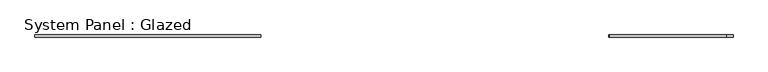
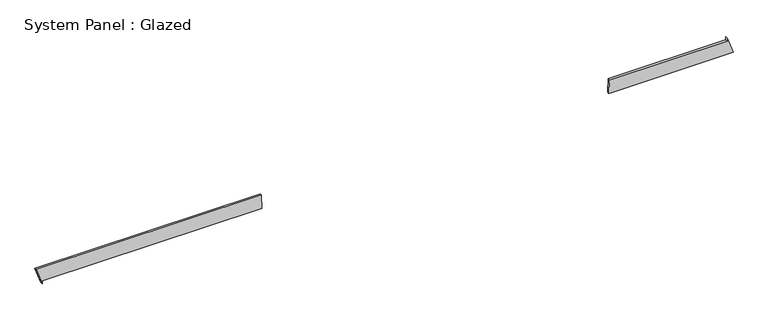
"""IFC4 building model written with IfcOpenShell, lengths in millimetres: plate geometry, System Panel : Glazed."""

import ifcopenshell
import ifcopenshell.guid

model = None  # the IFC model being written
_history = None  # IfcOwnerHistory: only IFC2X3 demands one
_inside = {}  # id of a spatial element -> (the spatial element, [elements in it])
_under = {}  # id of a project, library or spatial element -> (it, [spatial elements below it])
_declared = {}  # id of a project -> (the project, [libraries it declares])
_typed = {}  # id of a type object -> (the type object, [elements of that type])
_made_of = {}  # id of a material, layer set ... -> (it, [elements and type objects made of it])


def new_model(schema):
    """Start an empty IFC model of exactly this schema.

    Asked for "IFC4X3", IfcOpenShell would pick the latest addendum, in which some entities
    have other attributes; the version numbers below select the first issue.
    IFC2X3 requires an IfcOwnerHistory on every rooted entity: one is made here for all.
    """
    global model, _history
    if schema == "IFC4X3":
        model = ifcopenshell.file(schema_version=(4, 3, 0, 0))
    else:
        model = ifcopenshell.file(schema=schema)
    _inside.clear()
    _under.clear()
    _declared.clear()
    _typed.clear()
    _made_of.clear()
    _history = None
    if model.schema == "IFC2X3":
        org = make("IfcOrganization", Name="unknown")
        user = make(
            "IfcPersonAndOrganization",
            ThePerson=make("IfcPerson", FamilyName="unknown"),
            TheOrganization=org,
        )
        app = make(
            "IfcApplication",
            ApplicationDeveloper=org,
            Version="unknown",
            ApplicationFullName="unknown",
            ApplicationIdentifier="unknown",
        )
        _history = make(
            "IfcOwnerHistory",
            OwningUser=user,
            OwningApplication=app,
            ChangeAction="ADDED",
            CreationDate=0,
        )
    return model


def make(cls, **values):
    """One entity of the class cls with the attributes given. An attribute that is None is left unset."""
    return model.create_entity(
        cls, **{name: value for name, value in values.items() if value is not None}
    )


def rooted(cls, **values):
    """An entity with a GlobalId (a new one), such as an element, a storey or a relation."""
    return make(cls, GlobalId=ifcopenshell.guid.new(), OwnerHistory=_history, **values)


def si_unit(unit_type, name, prefix=None):
    """IfcSIUnit, for example si_unit("LENGTHUNIT", "METRE", prefix="MILLI")."""
    return make("IfcSIUnit", UnitType=unit_type, Prefix=prefix, Name=name)


def assignment(units):
    """IfcUnitAssignment: the units of a project."""
    return None if units is None else make("IfcUnitAssignment", Units=units)


def point(xyz):
    """IfcCartesianPoint."""
    return None if xyz is None else make("IfcCartesianPoint", Coordinates=xyz)


def direction(xyz):
    """IfcDirection."""
    return None if xyz is None else make("IfcDirection", DirectionRatios=xyz)


def frame(location, z_axis=None, x_axis=None):
    """IfcAxis2Placement3D, a coordinate frame: its origin and axes. An axis left out is left unset."""
    return make(
        "IfcAxis2Placement3D",
        Location=point(location),
        Axis=direction(z_axis),
        RefDirection=direction(x_axis),
    )


def origin():
    """The frame at (0, 0, 0) with its axes left unset."""
    return frame((0.0, 0.0, 0.0))


def place(relative_to, where):
    """IfcLocalPlacement: puts the frame where relative to a parent placement (None: the world)."""
    return make(
        "IfcLocalPlacement", PlacementRelTo=relative_to, RelativePlacement=where
    )


def context(
    kind, dimensions, precision=None, world=None, true_north=None, identifier=None
):
    """IfcGeometricRepresentationContext, for example the 3D "Model" context."""
    return make(
        "IfcGeometricRepresentationContext",
        ContextIdentifier=identifier,
        ContextType=kind,
        CoordinateSpaceDimension=dimensions,
        Precision=precision,
        WorldCoordinateSystem=world,
        TrueNorth=true_north,
    )


def project(units=None, contexts=None):
    """IfcProject with its units and contexts."""
    return rooted(
        "IfcProject",
        Name="project",
        RepresentationContexts=contexts,
        UnitsInContext=assignment(units),
    )


def spatial(cls, under=None, at=None, **own):
    """A site, building, storey or space (cls), placed at a placement, below another one or the project."""
    s = rooted(cls, ObjectPlacement=at, **own)
    if under is not None:
        _under.setdefault(under.id(), (under, []))[1].append(s)
    return s


def polyline(points):
    """IfcPolyline through the points."""
    return make("IfcPolyline", Points=[point(p) for p in points])


def outline(outer, holes=None, kind="AREA"):
    """IfcArbitraryClosedProfileDef: a profile drawn as a closed curve; with holes, ...WithVoids."""
    if holes is None:
        return make("IfcArbitraryClosedProfileDef", ProfileType=kind, OuterCurve=outer)
    return make(
        "IfcArbitraryProfileDefWithVoids",
        ProfileType=kind,
        OuterCurve=outer,
        InnerCurves=holes,
    )


def extrude(swept, where, along, depth):
    """IfcExtrudedAreaSolid: the profile swept, set in the frame where, extruded along a direction by depth."""
    return make(
        "IfcExtrudedAreaSolid",
        SweptArea=swept,
        Position=where,
        ExtrudedDirection=direction(along),
        Depth=depth,
    )


def shape(context_of_items, identifier, shape_type, items):
    """IfcShapeRepresentation: the items that make up one representation, for example the "Body"."""
    return make(
        "IfcShapeRepresentation",
        ContextOfItems=context_of_items,
        RepresentationIdentifier=identifier,
        RepresentationType=shape_type,
        Items=items,
    )


def source(mapping_origin, context_of_items, identifier, shape_type, items):
    """IfcRepresentationMap: a shape defined once, which mapped items show again and again."""
    return make(
        "IfcRepresentationMap",
        MappingOrigin=mapping_origin,
        MappedRepresentation=shape(context_of_items, identifier, shape_type, items),
    )


def transform(
    local_origin,
    x_axis=None,
    y_axis=None,
    z_axis=None,
    scale=None,
    scale2=None,
    scale3=None,
    uniform=True,
):
    """IfcCartesianTransformationOperator3D, or its non-uniform kind. x_axis, y_axis, z_axis: its Axis1, 2, 3."""
    if uniform:
        return make(
            "IfcCartesianTransformationOperator3D",
            Axis1=direction(x_axis),
            Axis2=direction(y_axis),
            LocalOrigin=point(local_origin),
            Scale=scale,
            Axis3=direction(z_axis),
        )
    return make(
        "IfcCartesianTransformationOperator3DnonUniform",
        Axis1=direction(x_axis),
        Axis2=direction(y_axis),
        LocalOrigin=point(local_origin),
        Scale=scale,
        Axis3=direction(z_axis),
        Scale2=scale2,
        Scale3=scale3,
    )


def mapped(mapping_source, mapping_target):
    """IfcMappedItem: shows the shape of a source again, moved by a transform."""
    return make(
        "IfcMappedItem", MappingSource=mapping_source, MappingTarget=mapping_target
    )


def made_of(thing, what):
    """Note that an element or type object is made of a material, layer set ...; save() writes the relation."""
    if what is not None:
        _made_of.setdefault(what.id(), (what, []))[1].append(thing)
    return thing


def element(
    cls,
    number,
    at=None,
    inside=None,
    cuts=None,
    type_object=None,
    material=None,
    context=None,
    identifier="Body",
    shape_type=None,
    held_by="IfcProductDefinitionShape",
    body=None,
    shapes=None,
    **own,
):
    """One element of the class cls, such as IfcWall. Its Tag is "e" and its number.

    at: its placement. inside: the storey or other place that contains it. cuts: it is an
    opening in that element (IfcRelVoidsElement). A single representation is given by context,
    identifier, shape_type and body (its items); several are given by shapes. held_by: the class
    of the entity that holds the representations. save() writes the other relations.
    """
    e = rooted(cls, Tag="e%d" % number, ObjectPlacement=at, **own)
    if body is not None:
        shapes = [shape(context, identifier, shape_type, body)]
    if shapes is not None:
        e.Representation = make(held_by, Representations=shapes)
    if inside is not None:
        _inside.setdefault(inside.id(), (inside, []))[1].append(e)
    if cuts is not None:
        rooted(
            "IfcRelVoidsElement", RelatingBuildingElement=cuts, RelatedOpeningElement=e
        )
    if type_object is not None:
        _typed.setdefault(type_object.id(), (type_object, []))[1].append(e)
    return made_of(e, material)


def aggregate(whole, parts):
    """IfcRelAggregates: a whole, such as a stair, and the parts it consists of."""
    return rooted("IfcRelAggregates", RelatingObject=whole, RelatedObjects=parts)


def save(model, path):
    """Write the relations noted so far, then the file.

    IfcRelAggregates (storeys below a building ...), IfcRelContainedInSpatialStructure (elements
    in a storey), IfcRelDefinesByType, IfcRelAssociatesMaterial and IfcRelDeclares: one each for
    every whole, place, type object, material and project.
    """
    for whole, parts in _under.values():
        aggregate(whole, parts)
    for where, things in _inside.values():
        rooted(
            "IfcRelContainedInSpatialStructure",
            RelatedElements=things,
            RelatingStructure=where,
        )
    for kind, things in _typed.values():
        rooted("IfcRelDefinesByType", RelatedObjects=things, RelatingType=kind)
    for what, things in _made_of.values():
        rooted("IfcRelAssociatesMaterial", RelatedObjects=things, RelatingMaterial=what)
    for by, libraries in _declared.values():
        rooted("IfcRelDeclares", RelatingContext=by, RelatedDefinitions=libraries)
    model.write(path)


def system_panel_glazed_22199b68(model_context):
    return source(origin(), model_context, "Body", "SweptSolid", [
        extrude(outline(polyline([(35.3553391, 2592.9093212), (35.3553391, 4027.1398136), (235.0472205, 3956.767991), (199.6918814, 3956.7680004), (199.6915206, 2596.4691848), (35.3553391, 2592.9093212)])), frame((0.0, -49.5, 0.0), z_axis=(0.0, 1.0, 0.0), x_axis=(0.0, 0.0, 1.0)), (0.0, 0.0, 1.0), 25.0),
        extrude(outline(polyline([(0.0, -3956.7629895), (35.3553391, -3956.7629895), (35.3553391, -1422.2011532), (199.6904543, -1424.1483538), (199.6897639, -4027.1398136), (0.0, -3956.7629895)])), frame((0.0, -49.5, 0.0), z_axis=(0.0, 1.0, 0.0), x_axis=(0.0, 0.0, 1.0)), (0.0, 0.0, 1.0), 25.0),
    ])


if __name__ == "__main__":
    model = new_model("IFC4")
    model_context = context("Model", 3, world=origin())
    ifc_project = project(units=[si_unit("LENGTHUNIT", "METRE", prefix="MILLI")], contexts=[model_context])
    site = spatial("IfcSite", under=ifc_project)
    building = spatial("IfcBuilding", under=site)
    placement = place(None, origin())
    system_panel_glazed_shape = system_panel_glazed_22199b68(model_context)
    element("IfcPlate", 1, ObjectType="System Panel : Glazed", at=placement, inside=building, context=model_context, shape_type="MappedRepresentation", body=[
        mapped(system_panel_glazed_shape, transform((0.0, 0.0, 0.0), x_axis=(1.0, 0.0, 0.0), y_axis=(0.0, 1.0, 0.0), z_axis=(0.0, 0.0, 1.0))),
    ])
    save(model, "model.ifc")

# Revit data of these elements
# Element 1 (IfcPlate, "System Panel : Glazed")
#   Materials on its faces: "Glass"
# Materials
#   "Glass": class "Glass", colour RGB 218 227 224, transparency 0.85, Description = "Soda Lime Glass", Cost = 0
